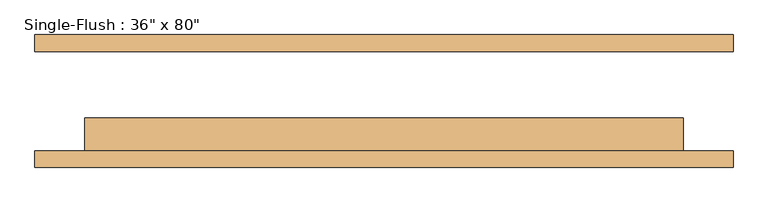
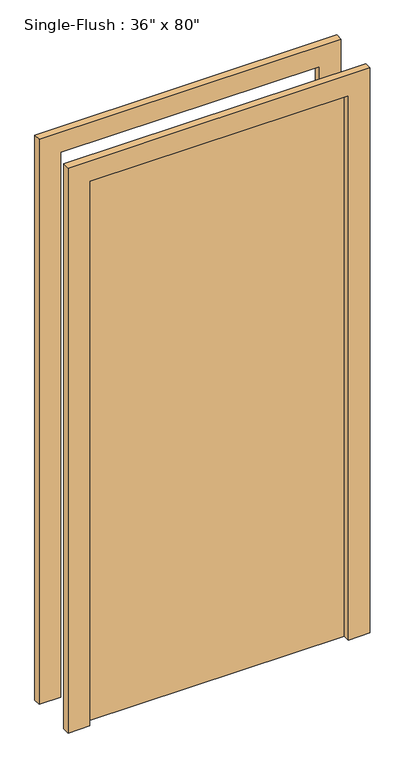
"""IFC4 building model written with IfcOpenShell, lengths in millimetres: door geometry."""

import ifcopenshell
import ifcopenshell.guid

model = None  # the IFC model being written
_history = None  # IfcOwnerHistory: only IFC2X3 demands one
_inside = {}  # id of a spatial element -> (the spatial element, [elements in it])
_under = {}  # id of a project, library or spatial element -> (it, [spatial elements below it])
_declared = {}  # id of a project -> (the project, [libraries it declares])
_typed = {}  # id of a type object -> (the type object, [elements of that type])
_made_of = {}  # id of a material, layer set ... -> (it, [elements and type objects made of it])


def new_model(schema):
    """Start an empty IFC model of exactly this schema.

    Asked for "IFC4X3", IfcOpenShell would pick the latest addendum, in which some entities
    have other attributes; the version numbers below select the first issue.
    IFC2X3 requires an IfcOwnerHistory on every rooted entity: one is made here for all.
    """
    global model, _history
    if schema == "IFC4X3":
        model = ifcopenshell.file(schema_version=(4, 3, 0, 0))
    else:
        model = ifcopenshell.file(schema=schema)
    _inside.clear()
    _under.clear()
    _declared.clear()
    _typed.clear()
    _made_of.clear()
    _history = None
    if model.schema == "IFC2X3":
        org = make("IfcOrganization", Name="unknown")
        user = make(
            "IfcPersonAndOrganization",
            ThePerson=make("IfcPerson", FamilyName="unknown"),
            TheOrganization=org,
        )
        app = make(
            "IfcApplication",
            ApplicationDeveloper=org,
            Version="unknown",
            ApplicationFullName="unknown",
            ApplicationIdentifier="unknown",
        )
        _history = make(
            "IfcOwnerHistory",
            OwningUser=user,
            OwningApplication=app,
            ChangeAction="ADDED",
            CreationDate=0,
        )
    return model


def make(cls, **values):
    """One entity of the class cls with the attributes given. An attribute that is None is left unset."""
    return model.create_entity(
        cls, **{name: value for name, value in values.items() if value is not None}
    )


def rooted(cls, **values):
    """An entity with a GlobalId (a new one), such as an element, a storey or a relation."""
    return make(cls, GlobalId=ifcopenshell.guid.new(), OwnerHistory=_history, **values)


def si_unit(unit_type, name, prefix=None):
    """IfcSIUnit, for example si_unit("LENGTHUNIT", "METRE", prefix="MILLI")."""
    return make("IfcSIUnit", UnitType=unit_type, Prefix=prefix, Name=name)


def assignment(units):
    """IfcUnitAssignment: the units of a project."""
    return None if units is None else make("IfcUnitAssignment", Units=units)


def point(xyz):
    """IfcCartesianPoint."""
    return None if xyz is None else make("IfcCartesianPoint", Coordinates=xyz)


def direction(xyz):
    """IfcDirection."""
    return None if xyz is None else make("IfcDirection", DirectionRatios=xyz)


def frame(location, z_axis=None, x_axis=None):
    """IfcAxis2Placement3D, a coordinate frame: its origin and axes. An axis left out is left unset."""
    return make(
        "IfcAxis2Placement3D",
        Location=point(location),
        Axis=direction(z_axis),
        RefDirection=direction(x_axis),
    )


def origin():
    """The frame at (0, 0, 0) with its axes left unset."""
    return frame((0.0, 0.0, 0.0))


def origin_with_axes():
    """The frame at (0, 0, 0) with the z axis (0, 0, 1) and the x axis (1, 0, 0) written out."""
    return frame((0.0, 0.0, 0.0), z_axis=(0.0, 0.0, 1.0), x_axis=(1.0, 0.0, 0.0))


def place(relative_to, where):
    """IfcLocalPlacement: puts the frame where relative to a parent placement (None: the world)."""
    return make(
        "IfcLocalPlacement", PlacementRelTo=relative_to, RelativePlacement=where
    )


def context(
    kind, dimensions, precision=None, world=None, true_north=None, identifier=None
):
    """IfcGeometricRepresentationContext, for example the 3D "Model" context."""
    return make(
        "IfcGeometricRepresentationContext",
        ContextIdentifier=identifier,
        ContextType=kind,
        CoordinateSpaceDimension=dimensions,
        Precision=precision,
        WorldCoordinateSystem=world,
        TrueNorth=true_north,
    )


def project(units=None, contexts=None):
    """IfcProject with its units and contexts."""
    return rooted(
        "IfcProject",
        Name="project",
        RepresentationContexts=contexts,
        UnitsInContext=assignment(units),
    )


def spatial(cls, under=None, at=None, **own):
    """A site, building, storey or space (cls), placed at a placement, below another one or the project."""
    s = rooted(cls, ObjectPlacement=at, **own)
    if under is not None:
        _under.setdefault(under.id(), (under, []))[1].append(s)
    return s


def polyline(points):
    """IfcPolyline through the points."""
    return make("IfcPolyline", Points=[point(p) for p in points])


def outline(outer, holes=None, kind="AREA"):
    """IfcArbitraryClosedProfileDef: a profile drawn as a closed curve; with holes, ...WithVoids."""
    if holes is None:
        return make("IfcArbitraryClosedProfileDef", ProfileType=kind, OuterCurve=outer)
    return make(
        "IfcArbitraryProfileDefWithVoids",
        ProfileType=kind,
        OuterCurve=outer,
        InnerCurves=holes,
    )


def extrude(swept, where, along, depth):
    """IfcExtrudedAreaSolid: the profile swept, set in the frame where, extruded along a direction by depth."""
    return make(
        "IfcExtrudedAreaSolid",
        SweptArea=swept,
        Position=where,
        ExtrudedDirection=direction(along),
        Depth=depth,
    )


def shape(context_of_items, identifier, shape_type, items):
    """IfcShapeRepresentation: the items that make up one representation, for example the "Body"."""
    return make(
        "IfcShapeRepresentation",
        ContextOfItems=context_of_items,
        RepresentationIdentifier=identifier,
        RepresentationType=shape_type,
        Items=items,
    )


def source(mapping_origin, context_of_items, identifier, shape_type, items):
    """IfcRepresentationMap: a shape defined once, which mapped items show again and again."""
    return make(
        "IfcRepresentationMap",
        MappingOrigin=mapping_origin,
        MappedRepresentation=shape(context_of_items, identifier, shape_type, items),
    )


def transform(
    local_origin,
    x_axis=None,
    y_axis=None,
    z_axis=None,
    scale=None,
    scale2=None,
    scale3=None,
    uniform=True,
):
    """IfcCartesianTransformationOperator3D, or its non-uniform kind. x_axis, y_axis, z_axis: its Axis1, 2, 3."""
    if uniform:
        return make(
            "IfcCartesianTransformationOperator3D",
            Axis1=direction(x_axis),
            Axis2=direction(y_axis),
            LocalOrigin=point(local_origin),
            Scale=scale,
            Axis3=direction(z_axis),
        )
    return make(
        "IfcCartesianTransformationOperator3DnonUniform",
        Axis1=direction(x_axis),
        Axis2=direction(y_axis),
        LocalOrigin=point(local_origin),
        Scale=scale,
        Axis3=direction(z_axis),
        Scale2=scale2,
        Scale3=scale3,
    )


def mapped(mapping_source, mapping_target):
    """IfcMappedItem: shows the shape of a source again, moved by a transform."""
    return make(
        "IfcMappedItem", MappingSource=mapping_source, MappingTarget=mapping_target
    )


def made_of(thing, what):
    """Note that an element or type object is made of a material, layer set ...; save() writes the relation."""
    if what is not None:
        _made_of.setdefault(what.id(), (what, []))[1].append(thing)
    return thing


def element(
    cls,
    number,
    at=None,
    inside=None,
    cuts=None,
    type_object=None,
    material=None,
    context=None,
    identifier="Body",
    shape_type=None,
    held_by="IfcProductDefinitionShape",
    body=None,
    shapes=None,
    **own,
):
    """One element of the class cls, such as IfcWall. Its Tag is "e" and its number.

    at: its placement. inside: the storey or other place that contains it. cuts: it is an
    opening in that element (IfcRelVoidsElement). A single representation is given by context,
    identifier, shape_type and body (its items); several are given by shapes. held_by: the class
    of the entity that holds the representations. save() writes the other relations.
    """
    e = rooted(cls, Tag="e%d" % number, ObjectPlacement=at, **own)
    if body is not None:
        shapes = [shape(context, identifier, shape_type, body)]
    if shapes is not None:
        e.Representation = make(held_by, Representations=shapes)
    if inside is not None:
        _inside.setdefault(inside.id(), (inside, []))[1].append(e)
    if cuts is not None:
        rooted(
            "IfcRelVoidsElement", RelatingBuildingElement=cuts, RelatedOpeningElement=e
        )
    if type_object is not None:
        _typed.setdefault(type_object.id(), (type_object, []))[1].append(e)
    return made_of(e, material)


def aggregate(whole, parts):
    """IfcRelAggregates: a whole, such as a stair, and the parts it consists of."""
    return rooted("IfcRelAggregates", RelatingObject=whole, RelatedObjects=parts)


def save(model, path):
    """Write the relations noted so far, then the file.

    IfcRelAggregates (storeys below a building ...), IfcRelContainedInSpatialStructure (elements
    in a storey), IfcRelDefinesByType, IfcRelAssociatesMaterial and IfcRelDeclares: one each for
    every whole, place, type object, material and project.
    """
    for whole, parts in _under.values():
        aggregate(whole, parts)
    for where, things in _inside.values():
        rooted(
            "IfcRelContainedInSpatialStructure",
            RelatedElements=things,
            RelatingStructure=where,
        )
    for kind, things in _typed.values():
        rooted("IfcRelDefinesByType", RelatedObjects=things, RelatingType=kind)
    for what, things in _made_of.values():
        rooted("IfcRelAssociatesMaterial", RelatedObjects=things, RelatingMaterial=what)
    for by, libraries in _declared.values():
        rooted("IfcRelDeclares", RelatingContext=by, RelatedDefinitions=libraries)
    model.write(path)


def door_2b0b55a0(model_context):
    return source(origin(), model_context, "Body", "SweptSolid", [
        extrude(outline(polyline([(2108.2, -533.4), (0.0, -533.4), (0.0, -457.2), (2032.0, -457.2), (2032.0, 457.2), (0.0, 457.2), (0.0, 533.4), (2108.2, 533.4), (2108.2, -533.4)])), frame((0.0, -101.6, 0.0), z_axis=(0.0, 1.0, 0.0), x_axis=(0.0, 0.0, 1.0)), (0.0, 0.0, 1.0), 25.4),
        extrude(outline(polyline([(2108.2, 533.4), (2108.2, -533.4), (0.0, -533.4), (0.0, -457.2), (2032.0, -457.2), (2032.0, 457.2), (0.0, 457.2), (0.0, 533.4), (2108.2, 533.4)])), frame((0.0, 76.2, 0.0), z_axis=(0.0, 1.0, 0.0), x_axis=(0.0, 0.0, 1.0)), (0.0, 0.0, 1.0), 25.4),
        extrude(outline(polyline([(457.2, -25.4), (457.2, -76.2), (-457.2, -76.2), (-457.2, -25.4), (457.2, -25.4)])), origin_with_axes(), (0.0, 0.0, 1.0), 2032.0),
    ])


if __name__ == "__main__":
    model = new_model("IFC4")
    model_context = context("Model", 3, world=origin())
    ifc_project = project(units=[si_unit("LENGTHUNIT", "METRE", prefix="MILLI")], contexts=[model_context])
    site = spatial("IfcSite", under=ifc_project)
    building = spatial("IfcBuilding", under=site)
    placement = place(None, origin())
    door_shape = door_2b0b55a0(model_context)
    element("IfcDoor", 1, ObjectType="Single-Flush : 36\" x 80\"", at=placement, inside=building, context=model_context, shape_type="MappedRepresentation", body=[
        mapped(door_shape, transform((0.0, 0.0, 0.0), x_axis=(1.0, 0.0, 0.0), y_axis=(0.0, 1.0, 0.0), z_axis=(0.0, 0.0, 1.0))),
    ])
    save(model, "model.ifc")

# Revit data of these elements
# Type "Single-Flush : 36\" x 80\""
#   Type Mark = "6"
#   Assembly Code = "C1020"
#   Thickness = 0' - 2"
#   Height = 6' - 8"
#   Trim Projection Ext = 0' - 1"
#   Trim Projection Int = 0' - 1"
#   Trim Width = 0' - 3"
#   Width = 3' - 0"
#   Door Material = Door - Panel
#   Frame Material = Door - Frame
#   Function = (empty or 0)
#   Wall Closure = (empty or 0)
# Element 1 (IfcDoor, "Single-Flush : 36\" x 80\"")
#   Materials on its faces: "Door - Frame", "Door - Panel"
# Materials
#   "Door - Panel": class "Wood", colour RGB 114 82 51, transparency 0
#   "Door - Frame": class "Miscellaneous", colour RGB 153 76 43, transparency 0
